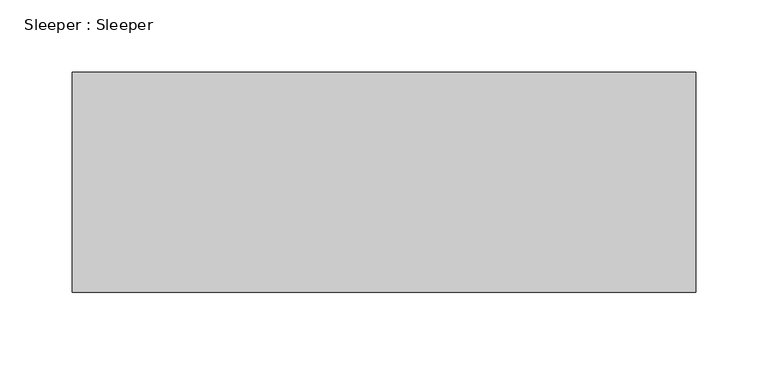
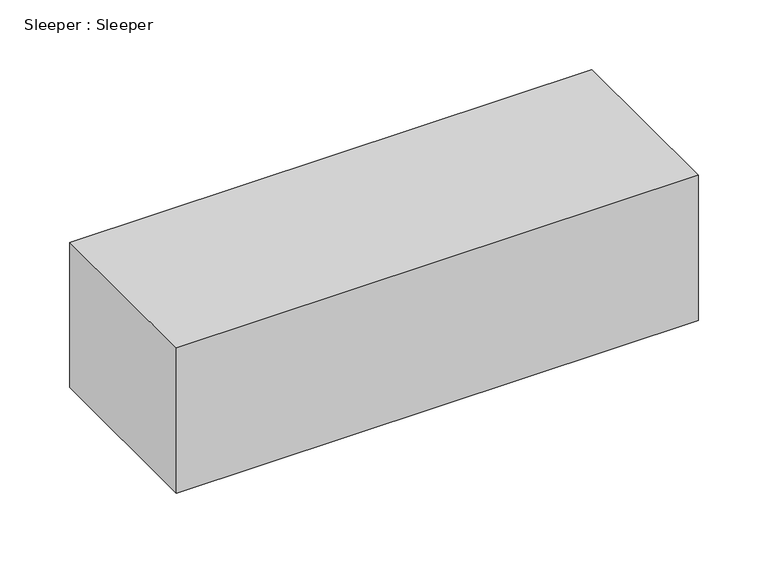
"""IFC4 building model written with IfcOpenShell, lengths in millimetres: proxy geometry, Sleeper : Sleeper."""

from ifc_helpers import new_model, si_unit, frame, origin, place, context, project, spatial, polyline, outline, extrude, source, transform, mapped, element, save


def sleeper_sleeper_7f78abd6(model_context):
    return source(origin(), model_context, "Body", "SweptSolid", [
        extrude(outline(polyline([(-9372.0566199, 9829.7531721), (-9803.8565956, 9829.7531721), (-9803.8565956, 9982.1531721), (-9372.0566199, 9982.1531721), (-9372.0566199, 9829.7531721)])), frame((0.0, 0.0, 39953.9745281), z_axis=(0.0, 0.0, 1.0), x_axis=(1.0, 0.0, 0.0)), (0.0, 0.0, 1.0), 126.9999929),
    ])


if __name__ == "__main__":
    model = new_model("IFC4")
    model_context = context("Model", 3, world=origin())
    ifc_project = project(units=[si_unit("LENGTHUNIT", "METRE", prefix="MILLI")], contexts=[model_context])
    site = spatial("IfcSite", under=ifc_project)
    building = spatial("IfcBuilding", under=site)
    placement = place(None, origin())
    sleeper_sleeper_shape = sleeper_sleeper_7f78abd6(model_context)
    element("IfcBuildingElementProxy", 1, Name="Sleeper : Sleeper", ObjectType="Sleeper : Sleeper", at=placement, inside=building, context=model_context, shape_type="MappedRepresentation", body=[
        mapped(sleeper_sleeper_shape, transform((0.0, 0.0, 0.0), x_axis=(1.0, 0.0, 0.0), y_axis=(0.0, 1.0, 0.0), z_axis=(0.0, 0.0, 1.0))),
    ])
    save(model, "model.ifc")

# Revit data of these elements
# Type "Sleeper : Sleeper"
#   NameOverride = "Sleeper"
# Element 1 (IfcBuildingElementProxy, "Sleeper : Sleeper")
#   Materials on its faces: "2X SLOPED SLEEPERS - SLOPE TO DRAINS"
# Materials
#   "2X SLOPED SLEEPERS - SLOPE TO DRAINS": class "Unassigned", colour RGB 234 198 178, transparency 0
